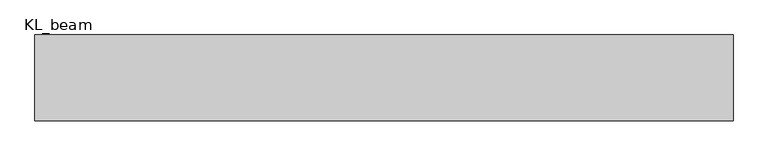
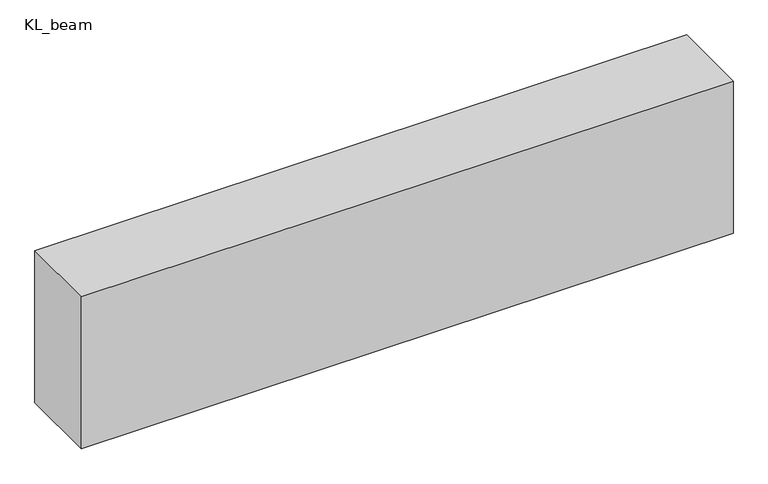
"""IFC4 building model written with IfcOpenShell, lengths in millimetres: beam geometry, 混凝土 - 矩形梁 : KL_beam."""

import ifcopenshell
import ifcopenshell.guid

model = None  # the IFC model being written
_history = None  # IfcOwnerHistory: only IFC2X3 demands one
_inside = {}  # id of a spatial element -> (the spatial element, [elements in it])
_under = {}  # id of a project, library or spatial element -> (it, [spatial elements below it])
_declared = {}  # id of a project -> (the project, [libraries it declares])
_typed = {}  # id of a type object -> (the type object, [elements of that type])
_made_of = {}  # id of a material, layer set ... -> (it, [elements and type objects made of it])


def new_model(schema):
    """Start an empty IFC model of exactly this schema.

    Asked for "IFC4X3", IfcOpenShell would pick the latest addendum, in which some entities
    have other attributes; the version numbers below select the first issue.
    IFC2X3 requires an IfcOwnerHistory on every rooted entity: one is made here for all.
    """
    global model, _history
    if schema == "IFC4X3":
        model = ifcopenshell.file(schema_version=(4, 3, 0, 0))
    else:
        model = ifcopenshell.file(schema=schema)
    _inside.clear()
    _under.clear()
    _declared.clear()
    _typed.clear()
    _made_of.clear()
    _history = None
    if model.schema == "IFC2X3":
        org = make("IfcOrganization", Name="unknown")
        user = make(
            "IfcPersonAndOrganization",
            ThePerson=make("IfcPerson", FamilyName="unknown"),
            TheOrganization=org,
        )
        app = make(
            "IfcApplication",
            ApplicationDeveloper=org,
            Version="unknown",
            ApplicationFullName="unknown",
            ApplicationIdentifier="unknown",
        )
        _history = make(
            "IfcOwnerHistory",
            OwningUser=user,
            OwningApplication=app,
            ChangeAction="ADDED",
            CreationDate=0,
        )
    return model


def make(cls, **values):
    """One entity of the class cls with the attributes given. An attribute that is None is left unset."""
    return model.create_entity(
        cls, **{name: value for name, value in values.items() if value is not None}
    )


def rooted(cls, **values):
    """An entity with a GlobalId (a new one), such as an element, a storey or a relation."""
    return make(cls, GlobalId=ifcopenshell.guid.new(), OwnerHistory=_history, **values)


def si_unit(unit_type, name, prefix=None):
    """IfcSIUnit, for example si_unit("LENGTHUNIT", "METRE", prefix="MILLI")."""
    return make("IfcSIUnit", UnitType=unit_type, Prefix=prefix, Name=name)


def assignment(units):
    """IfcUnitAssignment: the units of a project."""
    return None if units is None else make("IfcUnitAssignment", Units=units)


def point(xyz):
    """IfcCartesianPoint."""
    return None if xyz is None else make("IfcCartesianPoint", Coordinates=xyz)


def direction(xyz):
    """IfcDirection."""
    return None if xyz is None else make("IfcDirection", DirectionRatios=xyz)


def frame(location, z_axis=None, x_axis=None):
    """IfcAxis2Placement3D, a coordinate frame: its origin and axes. An axis left out is left unset."""
    return make(
        "IfcAxis2Placement3D",
        Location=point(location),
        Axis=direction(z_axis),
        RefDirection=direction(x_axis),
    )


def origin():
    """The frame at (0, 0, 0) with its axes left unset."""
    return frame((0.0, 0.0, 0.0))


def place(relative_to, where):
    """IfcLocalPlacement: puts the frame where relative to a parent placement (None: the world)."""
    return make(
        "IfcLocalPlacement", PlacementRelTo=relative_to, RelativePlacement=where
    )


def context(
    kind, dimensions, precision=None, world=None, true_north=None, identifier=None
):
    """IfcGeometricRepresentationContext, for example the 3D "Model" context."""
    return make(
        "IfcGeometricRepresentationContext",
        ContextIdentifier=identifier,
        ContextType=kind,
        CoordinateSpaceDimension=dimensions,
        Precision=precision,
        WorldCoordinateSystem=world,
        TrueNorth=true_north,
    )


def project(units=None, contexts=None):
    """IfcProject with its units and contexts."""
    return rooted(
        "IfcProject",
        Name="project",
        RepresentationContexts=contexts,
        UnitsInContext=assignment(units),
    )


def spatial(cls, under=None, at=None, **own):
    """A site, building, storey or space (cls), placed at a placement, below another one or the project."""
    s = rooted(cls, ObjectPlacement=at, **own)
    if under is not None:
        _under.setdefault(under.id(), (under, []))[1].append(s)
    return s


def polyline(points):
    """IfcPolyline through the points."""
    return make("IfcPolyline", Points=[point(p) for p in points])


def outline(outer, holes=None, kind="AREA"):
    """IfcArbitraryClosedProfileDef: a profile drawn as a closed curve; with holes, ...WithVoids."""
    if holes is None:
        return make("IfcArbitraryClosedProfileDef", ProfileType=kind, OuterCurve=outer)
    return make(
        "IfcArbitraryProfileDefWithVoids",
        ProfileType=kind,
        OuterCurve=outer,
        InnerCurves=holes,
    )


def extrude(swept, where, along, depth):
    """IfcExtrudedAreaSolid: the profile swept, set in the frame where, extruded along a direction by depth."""
    return make(
        "IfcExtrudedAreaSolid",
        SweptArea=swept,
        Position=where,
        ExtrudedDirection=direction(along),
        Depth=depth,
    )


def shape(context_of_items, identifier, shape_type, items):
    """IfcShapeRepresentation: the items that make up one representation, for example the "Body"."""
    return make(
        "IfcShapeRepresentation",
        ContextOfItems=context_of_items,
        RepresentationIdentifier=identifier,
        RepresentationType=shape_type,
        Items=items,
    )


def source(mapping_origin, context_of_items, identifier, shape_type, items):
    """IfcRepresentationMap: a shape defined once, which mapped items show again and again."""
    return make(
        "IfcRepresentationMap",
        MappingOrigin=mapping_origin,
        MappedRepresentation=shape(context_of_items, identifier, shape_type, items),
    )


def transform(
    local_origin,
    x_axis=None,
    y_axis=None,
    z_axis=None,
    scale=None,
    scale2=None,
    scale3=None,
    uniform=True,
):
    """IfcCartesianTransformationOperator3D, or its non-uniform kind. x_axis, y_axis, z_axis: its Axis1, 2, 3."""
    if uniform:
        return make(
            "IfcCartesianTransformationOperator3D",
            Axis1=direction(x_axis),
            Axis2=direction(y_axis),
            LocalOrigin=point(local_origin),
            Scale=scale,
            Axis3=direction(z_axis),
        )
    return make(
        "IfcCartesianTransformationOperator3DnonUniform",
        Axis1=direction(x_axis),
        Axis2=direction(y_axis),
        LocalOrigin=point(local_origin),
        Scale=scale,
        Axis3=direction(z_axis),
        Scale2=scale2,
        Scale3=scale3,
    )


def mapped(mapping_source, mapping_target):
    """IfcMappedItem: shows the shape of a source again, moved by a transform."""
    return make(
        "IfcMappedItem", MappingSource=mapping_source, MappingTarget=mapping_target
    )


def made_of(thing, what):
    """Note that an element or type object is made of a material, layer set ...; save() writes the relation."""
    if what is not None:
        _made_of.setdefault(what.id(), (what, []))[1].append(thing)
    return thing


def element(
    cls,
    number,
    at=None,
    inside=None,
    cuts=None,
    type_object=None,
    material=None,
    context=None,
    identifier="Body",
    shape_type=None,
    held_by="IfcProductDefinitionShape",
    body=None,
    shapes=None,
    **own,
):
    """One element of the class cls, such as IfcWall. Its Tag is "e" and its number.

    at: its placement. inside: the storey or other place that contains it. cuts: it is an
    opening in that element (IfcRelVoidsElement). A single representation is given by context,
    identifier, shape_type and body (its items); several are given by shapes. held_by: the class
    of the entity that holds the representations. save() writes the other relations.
    """
    e = rooted(cls, Tag="e%d" % number, ObjectPlacement=at, **own)
    if body is not None:
        shapes = [shape(context, identifier, shape_type, body)]
    if shapes is not None:
        e.Representation = make(held_by, Representations=shapes)
    if inside is not None:
        _inside.setdefault(inside.id(), (inside, []))[1].append(e)
    if cuts is not None:
        rooted(
            "IfcRelVoidsElement", RelatingBuildingElement=cuts, RelatedOpeningElement=e
        )
    if type_object is not None:
        _typed.setdefault(type_object.id(), (type_object, []))[1].append(e)
    return made_of(e, material)


def aggregate(whole, parts):
    """IfcRelAggregates: a whole, such as a stair, and the parts it consists of."""
    return rooted("IfcRelAggregates", RelatingObject=whole, RelatedObjects=parts)


def save(model, path):
    """Write the relations noted so far, then the file.

    IfcRelAggregates (storeys below a building ...), IfcRelContainedInSpatialStructure (elements
    in a storey), IfcRelDefinesByType, IfcRelAssociatesMaterial and IfcRelDeclares: one each for
    every whole, place, type object, material and project.
    """
    for whole, parts in _under.values():
        aggregate(whole, parts)
    for where, things in _inside.values():
        rooted(
            "IfcRelContainedInSpatialStructure",
            RelatedElements=things,
            RelatingStructure=where,
        )
    for kind, things in _typed.values():
        rooted("IfcRelDefinesByType", RelatedObjects=things, RelatingType=kind)
    for what, things in _made_of.values():
        rooted("IfcRelAssociatesMaterial", RelatedObjects=things, RelatingMaterial=what)
    for by, libraries in _declared.values():
        rooted("IfcRelDeclares", RelatingContext=by, RelatedDefinitions=libraries)
    model.write(path)


def kl_beam_b02ec389(model_context):
    return source(origin(), model_context, "Body", "SweptSolid", [
        extrude(outline(polyline([(1622.0, 200.0), (1622.0, -200.0), (-1622.0, -200.0), (-1622.0, 200.0), (1622.0, 200.0)])), frame((0.0, 0.0, -400.0), z_axis=(0.0, 0.0, 1.0), x_axis=(1.0, 0.0, 0.0)), (0.0, 0.0, 1.0), 800.0),
    ])


if __name__ == "__main__":
    model = new_model("IFC4")
    model_context = context("Model", 3, world=origin())
    ifc_project = project(units=[si_unit("LENGTHUNIT", "METRE", prefix="MILLI")], contexts=[model_context])
    site = spatial("IfcSite", under=ifc_project)
    building = spatial("IfcBuilding", under=site)
    placement = place(None, origin())
    kl_beam_shape = kl_beam_b02ec389(model_context)
    element("IfcBeam", 1, ObjectType="混凝土 - 矩形梁 : KL_beam", at=placement, inside=building, context=model_context, shape_type="MappedRepresentation", body=[
        mapped(kl_beam_shape, transform((0.0, 0.0, 0.0), x_axis=(1.0, 0.0, 0.0), y_axis=(0.0, 1.0, 0.0), z_axis=(0.0, 0.0, 1.0))),
    ])
    save(model, "model.ifc")

# Revit data of these elements
# Type "混凝土 - 矩形梁 : KL_beam"
#   Length [instance default] = 1524 mm
#   b = 400 mm
#   h = 800 mm
#   Structural Material [instance default] = 混凝土 - 现场浇注混凝土
#   Assembly Code = ""
# Element 1 (IfcBeam, "混凝土 - 矩形梁 : KL_beam")
#   Structural Material = none
# Materials
#   "混凝土 - 现场浇注混凝土": class "混凝土", colour RGB 192 192 192, transparency 0
